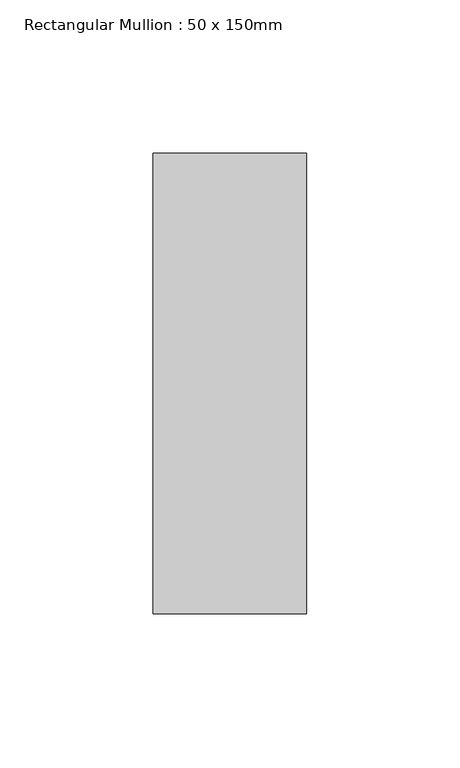
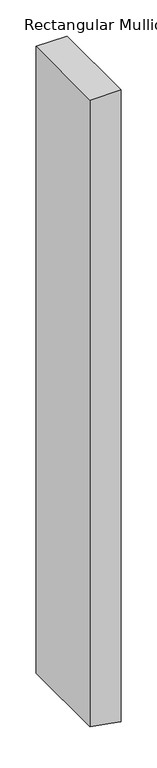
"""IFC4 building model written with IfcOpenShell, lengths in millimetres: member geometry, Rectangular Mullion : 50 x 150mm."""

from ifc_helpers import new_model, si_unit, frame, origin, place, context, project, spatial, polyline, outline, extrude, source, transform, mapped, element, save


def rectangular_mullion_50_x_150mm_576c40ba(model_context):
    return source(origin(), model_context, "Body", "SweptSolid", [
        extrude(outline(polyline([(0.0, 25.0), (0.0, -25.0), (-1061.2677449, -25.0), (-1066.4413909, 4.3412044), (-1070.084094, 25.0), (0.0, 25.0)])), frame((0.0, -75.0, 0.0), z_axis=(0.0, 1.0, 0.0), x_axis=(0.0, 0.0, 1.0)), (0.0, 0.0, 1.0), 150.0),
    ])


if __name__ == "__main__":
    model = new_model("IFC4")
    model_context = context("Model", 3, world=origin())
    ifc_project = project(units=[si_unit("LENGTHUNIT", "METRE", prefix="MILLI")], contexts=[model_context])
    site = spatial("IfcSite", under=ifc_project)
    building = spatial("IfcBuilding", under=site)
    placement = place(None, origin())
    rectangular_mullion_50_x_150mm_shape = rectangular_mullion_50_x_150mm_576c40ba(model_context)
    element("IfcMember", 1, ObjectType="Rectangular Mullion : 50 x 150mm", at=placement, inside=building, context=model_context, shape_type="MappedRepresentation", body=[
        mapped(rectangular_mullion_50_x_150mm_shape, transform((0.0, 0.0, 0.0), x_axis=(1.0, 0.0, 0.0), y_axis=(0.0, 1.0, 0.0), z_axis=(0.0, 0.0, 1.0))),
    ])
    save(model, "model.ifc")

# Revit data of these elements
# Type "Rectangular Mullion : 50 x 150mm"
#   built-in parameter 1007304 = 0.492126 (stored number, unit not read)
#   built-in parameter 1007301 = 0.082021 (stored number, unit not read)
#   built-in parameter 1007300 = 0.082021 (stored number, unit not read)
# Element 1 (IfcMember, "Rectangular Mullion : 50 x 150mm")
#   Materials on its faces: "Aluminium"
# Materials
#   "Aluminium": class "Metal", colour RGB 247 247 247, transparency 0, Description = "Aluminium 6061", Cost = 0
